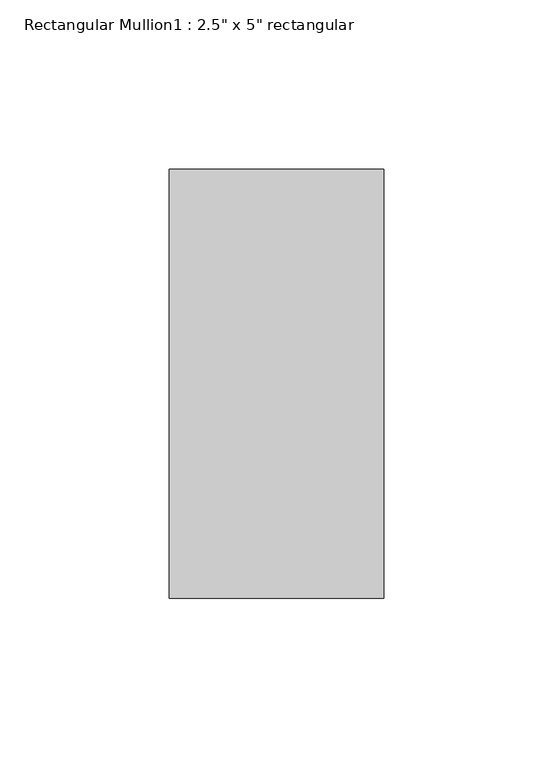
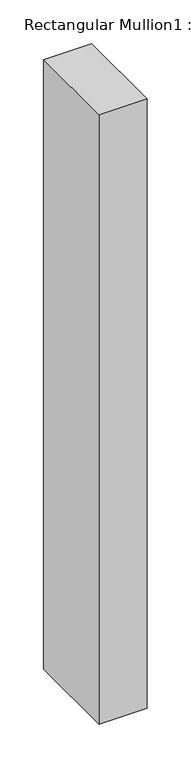
"""IFC4 building model written with IfcOpenShell, lengths in millimetres: member geometry."""

from ifc_helpers import new_model, si_unit, frame, origin, place, context, project, spatial, polyline, outline, extrude, source, transform, mapped, element, save


def member_7db1855a(model_context):
    return source(origin(), model_context, "Body", "SweptSolid", [
        extrude(outline(polyline([(31.75, 63.5), (31.75, -63.5), (-31.75, -63.5), (-31.75, 63.5), (31.75, 63.5)])), frame((0.0, 0.0, -850.9), z_axis=(0.0, 0.0, 1.0), x_axis=(1.0, 0.0, 0.0)), (0.0, 0.0, 1.0), 850.9),
    ])


if __name__ == "__main__":
    model = new_model("IFC4")
    model_context = context("Model", 3, world=origin())
    ifc_project = project(units=[si_unit("LENGTHUNIT", "METRE", prefix="MILLI")], contexts=[model_context])
    site = spatial("IfcSite", under=ifc_project)
    building = spatial("IfcBuilding", under=site)
    placement = place(None, origin())
    member_shape = member_7db1855a(model_context)
    element("IfcMember", 1, ObjectType="Rectangular Mullion1 : 2.5\" x 5\" rectangular", at=placement, inside=building, context=model_context, shape_type="MappedRepresentation", body=[
        mapped(member_shape, transform((0.0, 0.0, 0.0), x_axis=(1.0, 0.0, 0.0), y_axis=(0.0, 1.0, 0.0), z_axis=(0.0, 0.0, 1.0))),
    ])
    save(model, "model.ifc")

# Revit data of these elements
# Type "Rectangular Mullion1 : 2.5\" x 5\" rectangular"
#   built-in parameter 1007304 = 0.416667 (stored number, unit not read)
#   built-in parameter 1007301 = 0.104167 (stored number, unit not read)
#   built-in parameter 1007300 = 0.104167 (stored number, unit not read)
# Element 1 (IfcMember, "Rectangular Mullion1 : 2.5\" x 5\" rectangular")
#   Materials on its faces: "support-frame"
# Materials
#   "support-frame": class "Unassigned", colour RGB 233 233 233, transparency 0, Cost = 0
